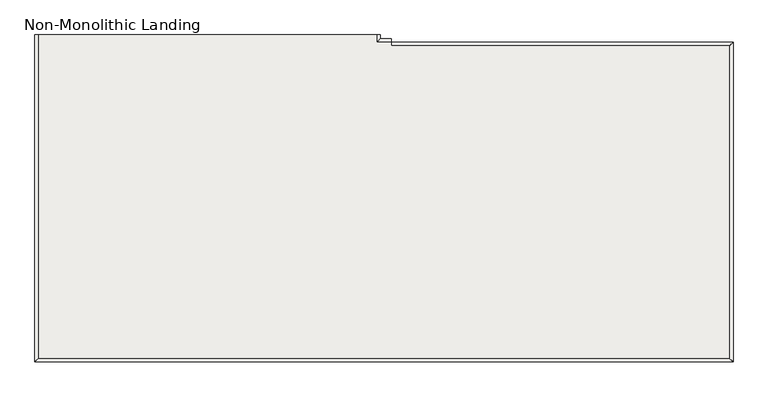
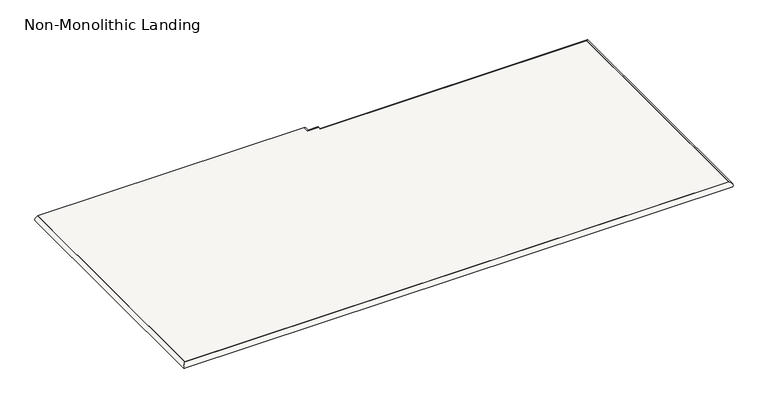
"""IFC4 building model written with IfcOpenShell, lengths in millimetres: slab geometry, Non-Monolithic Landing."""

from ifc_helpers import new_model, si_unit, frame, origin, place, context, project, spatial, circle_curve, ellipse_curve, faceted_brep, source, transform, mapped, element, save
from ifc_brep_helpers import plane_surface, cylinder_surface, advanced_brep


def non_monolithic_landing_0e10eb4c(model_context):
    return source(origin(), model_context, "Body", "SolidModel", [
        faceted_brep([(28388.4620052, 3855.5043237, 1400.175), (27220.0620052, 3855.5043237, 1400.175), (27220.0620052, 3868.2043237, 1400.175), (27169.2620052, 3868.2043237, 1400.175), (27169.2620052, 3893.6043237, 1400.175), (26000.8620052, 3893.6043237, 1400.175), (26000.8620052, 3868.2043237, 1400.175), (26000.8620052, 2776.0043237, 1400.175), (28388.4620052, 2776.0043237, 1400.175), (28388.4620052, 3855.5043237, 1374.775), (28388.4620052, 2776.0043237, 1374.775), (26000.8620052, 2776.0043237, 1374.775), (26000.8620052, 3868.2043237, 1374.775), (26000.8620052, 3893.6043237, 1374.775), (27169.2620052, 3893.6043237, 1374.775), (27169.2620052, 3868.2043237, 1374.775), (27220.0620052, 3868.2043237, 1374.775), (27220.0620052, 3855.5043237, 1374.775)], [[[0, 1, 2, 3, 4, 5, 6, 7, 8]], [[9, 10, 11, 12, 13, 14, 15, 16, 17]], [[1, 0, 9, 17]], [[2, 1, 17, 16]], [[3, 2, 16, 15]], [[4, 3, 15, 14]], [[5, 4, 14, 13]], [[6, 5, 13, 12]], [[7, 6, 12, 11]], [[8, 7, 11, 10]], [[0, 8, 10, 9]]]),
        advanced_brep(
        [(27169.2620052, 3893.6043237, 1400.175), (27169.2620052, 3893.6043237, 1374.775), (27169.2620052, 3868.2043237, 1400.175), (27169.2620052, 3868.2043237, 1374.775), (27220.0620052, 3868.2043237, 1400.175), (27220.0620052, 3868.2043237, 1374.775)],
        [
            (0, 1, circle_curve(frame((27169.2620052, 3893.6043237, 1387.475), z_axis=(0.0, 1.0, 0.0), x_axis=(-1.0, 0.0, 0.0)), 12.7)),
            (1, 0),
            (0, 2),
            (2, 3, ellipse_curve(frame((27169.2620052, 3868.2043237, 1387.475), z_axis=(-0.7071067811866013, 0.7071067811864937, 0.0), x_axis=(0.7071067811864937, 0.7071067811866013, 0.0)), 17.9605122, 12.7)),
            (3, 1),
            (3, 2),
            (4, 5),
            (5, 4, circle_curve(frame((27220.0620052, 3868.2043237, 1387.475), z_axis=(1.0, 0.0, 0.0), x_axis=(0.0, -1.0, 0.0)), 12.7)),
            (2, 4),
            (5, 3),
        ],
        [
            plane_surface(frame((27169.2620052, 3893.6043237, 1400.175), z_axis=(0.0, 1.0, 0.0), x_axis=(0.0, 0.0, 1.0))),
            cylinder_surface(frame((27169.2620052, 3893.6043237, 1387.475), z_axis=(0.0, 1.0, 0.0), x_axis=(-1.0, 0.0, 0.0)), 12.7),
            plane_surface(frame((27169.2620052, 3893.6043237, 1374.775), z_axis=(-1.0, 0.0, 0.0), x_axis=(0.0, -1.0, 0.0))),
            plane_surface(frame((27220.0620052, 3868.2043237, 1374.775), z_axis=(1.0, 0.0, 0.0), x_axis=(0.0, 1.0, 0.0))),
            cylinder_surface(frame((27169.2620052, 3868.2043237, 1387.475), z_axis=(-1.0, 0.0, 0.0), x_axis=(0.0, -1.0, 0.0)), 12.7),
            plane_surface(frame((27169.2620052, 3868.2043237, 1374.775), z_axis=(0.0, -1.0, 0.0), x_axis=(1.0, 0.0, 0.0))),
        ],
        [
            (0, [[1, 2]]),
            (1, [[-1, 3, 4, 5]]),
            (2, [[-2, -5, 6, -3]]),
            (3, [[7, 8]]),
            (4, [[-4, 9, -8, 10]]),
            (5, [[-6, -10, -7, -9]]),
        ],
    ),
        advanced_brep(
        [(27220.0620052, 3855.5043237, 1400.175), (27220.0620052, 3855.5043237, 1374.775), (28388.4620052, 3855.5043237, 1400.175), (28388.4620052, 3855.5043237, 1374.775), (28388.4620052, 2776.0043237, 1400.175), (28388.4620052, 2776.0043237, 1374.775), (26000.8620052, 2776.0043237, 1400.175), (26000.8620052, 2776.0043237, 1374.775), (26000.8620052, 3893.6043237, 1400.175), (26000.8620052, 3893.6043237, 1374.775)],
        [
            (0, 1, circle_curve(frame((27220.0620052, 3855.5043237, 1387.475), z_axis=(-1.0, 0.0, 0.0), x_axis=(0.0, -1.0, 0.0)), 12.7)),
            (1, 0),
            (0, 2),
            (2, 3, ellipse_curve(frame((28388.4620052, 3855.5043237, 1387.475), z_axis=(-0.707106781186558, 0.7071067811865371, 0.0), x_axis=(-0.707106781186537, -0.707106781186558, 0.0)), 17.9605122, 12.7)),
            (3, 1),
            (3, 2),
            (2, 4),
            (4, 5, ellipse_curve(frame((28388.4620052, 2776.0043237, 1387.475), z_axis=(0.707106781186543, 0.707106781186552, 0.0), x_axis=(-0.7071067811865519, 0.707106781186543, 0.0)), 17.9605122, 12.7)),
            (5, 3),
            (5, 4),
            (4, 6),
            (6, 7, ellipse_curve(frame((26000.8620052, 2776.0043237, 1387.475), z_axis=(0.7071067811865408, -0.7071067811865541, 0.0), x_axis=(0.7071067811865543, 0.7071067811865407, 0.0)), 17.9605122, 12.7)),
            (7, 5),
            (7, 6),
            (8, 9),
            (9, 8, circle_curve(frame((26000.8620052, 3893.6043237, 1387.475), z_axis=(0.0, 1.0, 0.0), x_axis=(1.0, 0.0, 0.0)), 12.7)),
            (6, 8),
            (9, 7),
        ],
        [
            plane_surface(frame((27220.0620052, 3855.5043237, 1374.775), z_axis=(-1.0, 0.0, 0.0), x_axis=(0.0, 1.0, 0.0))),
            cylinder_surface(frame((27220.0620052, 3855.5043237, 1387.475), z_axis=(-1.0, 0.0, 0.0), x_axis=(0.0, -1.0, 0.0)), 12.7),
            plane_surface(frame((27220.0620052, 3855.5043237, 1374.775), z_axis=(0.0, -1.0, 0.0), x_axis=(1.0, 0.0, 0.0))),
            cylinder_surface(frame((28388.4620052, 3855.5043237, 1387.475), z_axis=(0.0, 1.0, 0.0), x_axis=(-1.0, 0.0, 0.0)), 12.7),
            plane_surface(frame((28388.4620052, 3855.5043237, 1374.775), z_axis=(-1.0, 0.0, 0.0), x_axis=(0.0, -1.0, 0.0))),
            cylinder_surface(frame((28388.4620052, 2776.0043237, 1387.475), z_axis=(1.0, 0.0, 0.0), x_axis=(0.0, 1.0, 0.0)), 12.7),
            plane_surface(frame((28388.4620052, 2776.0043237, 1374.775), z_axis=(0.0, 1.0, 0.0), x_axis=(-1.0, 0.0, 0.0))),
            plane_surface(frame((26000.8620052, 3893.6043237, 1400.175), z_axis=(0.0, 1.0, 0.0), x_axis=(0.0, 0.0, 1.0))),
            cylinder_surface(frame((26000.8620052, 2776.0043237, 1387.475), z_axis=(0.0, -1.0, 0.0), x_axis=(1.0, 0.0, 0.0)), 12.7),
            plane_surface(frame((26000.8620052, 2776.0043237, 1374.775), z_axis=(1.0, 0.0, 0.0), x_axis=(0.0, 1.0, 0.0))),
        ],
        [
            (0, [[1, 2]]),
            (1, [[-1, 3, 4, 5]]),
            (2, [[-2, -5, 6, -3]]),
            (3, [[-4, 7, 8, 9]]),
            (4, [[-6, -9, 10, -7]]),
            (5, [[-8, 11, 12, 13]]),
            (6, [[-10, -13, 14, -11]]),
            (7, [[15, 16]]),
            (8, [[-12, 17, -16, 18]]),
            (9, [[-14, -18, -15, -17]]),
        ],
    ),
    ])


if __name__ == "__main__":
    model = new_model("IFC4")
    model_context = context("Model", 3, world=origin())
    ifc_project = project(units=[si_unit("LENGTHUNIT", "METRE", prefix="MILLI")], contexts=[model_context])
    site = spatial("IfcSite", under=ifc_project)
    building = spatial("IfcBuilding", under=site)
    placement = place(None, origin())
    non_monolithic_landing_shape = non_monolithic_landing_0e10eb4c(model_context)
    element("IfcSlab", 1, ObjectType="Non-Monolithic Landing", at=placement, inside=building, context=model_context, shape_type="MappedRepresentation", body=[
        mapped(non_monolithic_landing_shape, transform((0.0, 0.0, 0.0), x_axis=(1.0, 0.0, 0.0), y_axis=(0.0, 1.0, 0.0), z_axis=(0.0, 0.0, 1.0))),
    ])
    save(model, "model.ifc")

# Revit data of these elements
# Element 1 (IfcSlab, "Non-Monolithic Landing")
#   Materials on its faces: "FINISH T.B.D."
# Materials
#   "FINISH T.B.D.": class "Generic", colour RGB 227 188 136, transparency 0, Cost = 0
